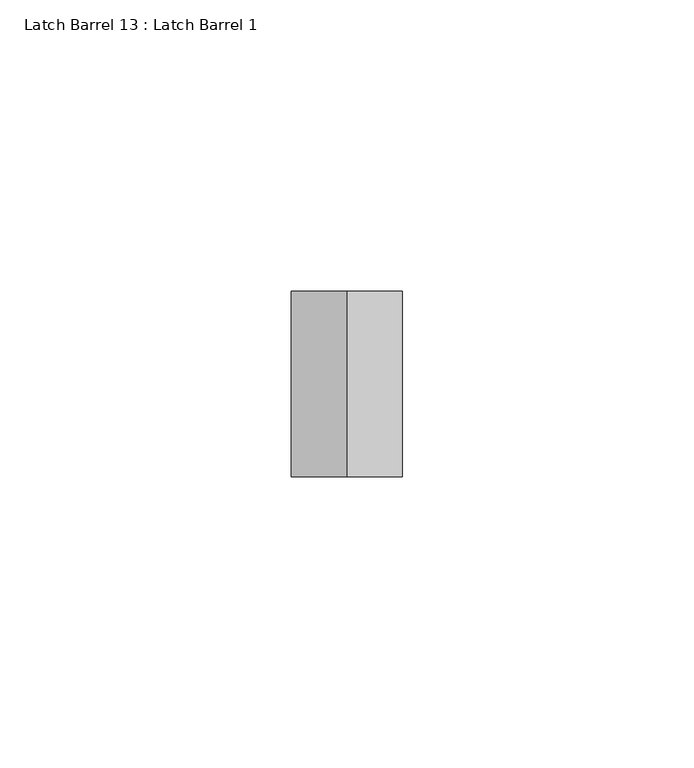
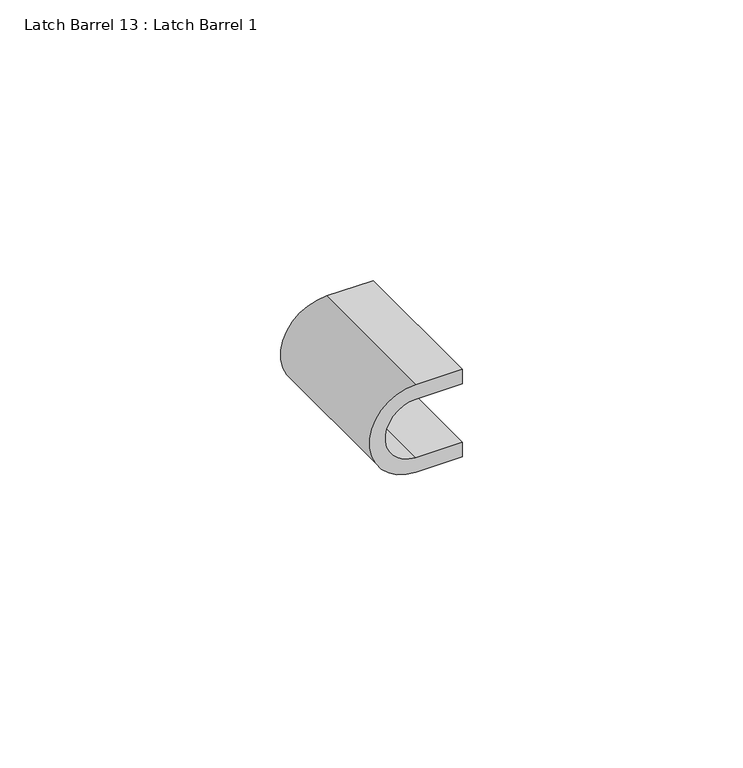
"""IFC4 building model written with IfcOpenShell, lengths in millimetres: proxy geometry, Latch Barrel 13 : Latch Barrel 1."""

from ifc_helpers import new_model, si_unit, point, frame, frame_2d, origin, place, context, project, spatial, polyline, circle_curve, trimmed, segment, composite_curve, outline, extrude, source, transform, mapped, element, save


def latch_barrel_13_latch_barrel_1_8cc6a647(model_context):
    return source(origin(), model_context, "Body", "SweptSolid", [
        extrude(outline(composite_curve([segment(trimmed(circle_curve(frame_2d((1066.8, 587312.7185739)), 6.35), [point((1060.45, 587312.7185739))], [point((1073.15, 587312.7185739))], True, "CARTESIAN"), True, "CONTINUOUS"), segment(polyline([(1073.15, 587312.7185739), (1073.15, 587322.2435739), (1076.325, 587322.2435739), (1076.325, 587312.7185739)]), True, "CONTINUOUS"), segment(trimmed(circle_curve(frame_2d((1066.8, 587312.7185739)), 9.525), [point((1076.325, 587312.7185739))], [point((1057.275, 587312.7185739))], False, "CARTESIAN"), True, "CONTINUOUS"), segment(polyline([(1057.275, 587312.7185739), (1057.275, 587322.2435739), (1060.45, 587322.2435739), (1060.45, 587312.7185739)]), True, "CONTINUOUS")], self_intersect=False)), frame((0.0, -532839.3663841, 0.0), z_axis=(0.0, 1.0, 0.0), x_axis=(0.0, 0.0, 1.0)), (0.0, 0.0, 1.0), 31.75),
    ])


if __name__ == "__main__":
    model = new_model("IFC4")
    model_context = context("Model", 3, world=origin())
    ifc_project = project(units=[si_unit("LENGTHUNIT", "METRE", prefix="MILLI")], contexts=[model_context])
    site = spatial("IfcSite", under=ifc_project)
    building = spatial("IfcBuilding", under=site)
    placement = place(None, origin())
    latch_barrel_13_latch_barrel_1_shape = latch_barrel_13_latch_barrel_1_8cc6a647(model_context)
    element("IfcBuildingElementProxy", 1, Name="Latch Barrel 13 : Latch Barrel 1", ObjectType="Latch Barrel 13 : Latch Barrel 1", at=placement, inside=building, context=model_context, shape_type="MappedRepresentation", body=[
        mapped(latch_barrel_13_latch_barrel_1_shape, transform((0.0, 0.0, 0.0), x_axis=(1.0, 0.0, 0.0), y_axis=(0.0, 1.0, 0.0), z_axis=(0.0, 0.0, 1.0))),
    ])
    save(model, "model.ifc")

# Revit data of these elements
# Element 1 (IfcBuildingElementProxy, "Latch Barrel 13 : Latch Barrel 1")
#   Materials on its faces: "GALV. GATE LATCH"
# Materials
#   "GALV. GATE LATCH": class "Metal", colour RGB 189 187 185, transparency 0, Description = "Carbon steel", Cost = 0
